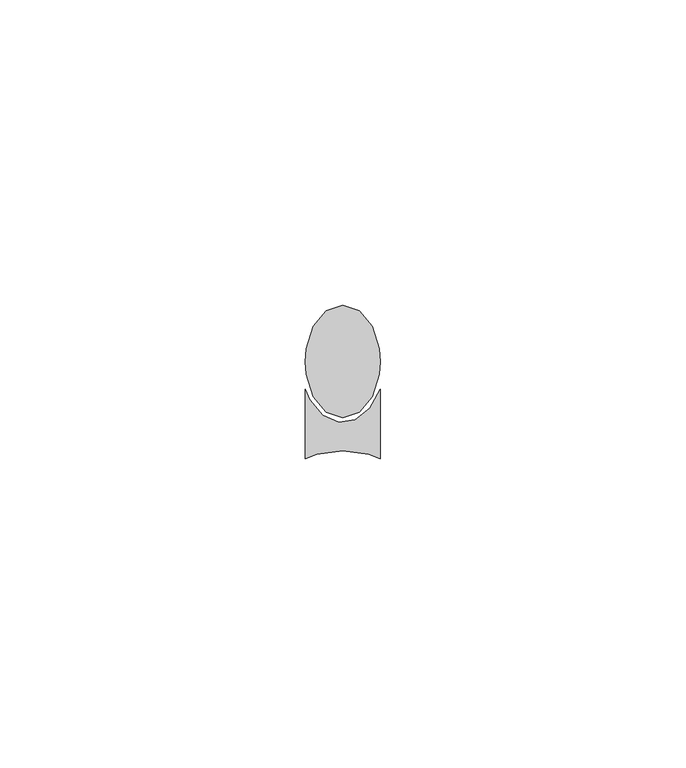
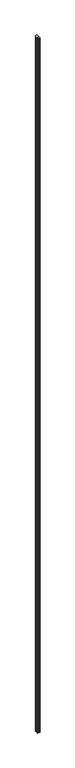
"""IFC4 building model written with IfcOpenShell, lengths in millimetres: proxy geometry, Generic Models 11:Generic Models 1:306267:Generic Models 1:306267 : Generic Models 11:Generic Models 1:306267:300405:Generic Models 1:306267:Generic Models 1:306267 : Generic Models 11:Generic Models 1:306267:300405 : Generic Models 11:Generic Models 1:306267:Generic Models 1:306267 : Generic Models 11:Generic Models 1:306267:300405:11 : Generic Models 11:Generic Models 1:306267:Generic Models 1:306267 : Generic Models 11:Generic Models 1:306267:300405:Generic Models 1:306267:Generic Models 1:306267 : Generic Models 11:Generic Models 1:306267:300405 : Generic Models 11:Generic Models 1:306267:Generic Models 1:306267 : Generic Models 11:Generic Models 1:306267:300405:300182."""

from ifc_helpers import new_model, si_unit, frame, origin, place, context, project, spatial, polyline, outline, extrude, source, transform, mapped, element, save


def generic_models_d67150ab(model_context):
    return source(origin(), model_context, "Body", "SweptSolid", [
        extrude(outline(polyline([(592759.9026632, -579084.0975007), (592755.6213645, -579083.4896058), (592751.3400657, -579084.0975007), (592749.468505, -579084.8288841), (592749.468505, -579073.4570585), (592750.2171531, -579075.1242043), (592752.3168487, -579077.6620411), (592754.9335054, -579078.8254713), (592757.6577712, -579078.4324869), (592760.0634599, -579076.5445668), (592761.7742239, -579073.4570585), (592761.7742239, -579084.8288841), (592759.9026632, -579084.0975007)])), frame((0.0, 0.0, 31.75), z_axis=(0.0, 0.0, 1.0), x_axis=(1.0, 0.0, 0.0)), (0.0, 0.0, 1.0), 3663.95),
        extrude(outline(polyline([(592752.9517388, -579077.1918668), (592750.8108652, -579074.6309323), (592749.62277, -579070.9302746), (592749.468505, -579068.8765646), (592749.62277, -579066.8228545), (592750.8108652, -579063.1221968), (592752.9517388, -579060.5612623), (592755.6213645, -579059.6472753), (592758.2909901, -579060.5612623), (592760.4318637, -579063.1221968), (592761.6199589, -579066.8228545), (592761.7742239, -579068.8765646), (592761.6199589, -579070.9302746), (592760.4318637, -579074.6309323), (592758.2909901, -579077.1918668), (592755.6213645, -579078.1058538), (592752.9517388, -579077.1918668)])), frame((0.0, 0.0, 31.75), z_axis=(0.0, 0.0, 1.0), x_axis=(1.0, 0.0, 0.0)), (0.0, 0.0, 1.0), 3663.95),
    ])


if __name__ == "__main__":
    model = new_model("IFC4")
    model_context = context("Model", 3, world=origin())
    ifc_project = project(units=[si_unit("LENGTHUNIT", "METRE", prefix="MILLI")], contexts=[model_context])
    site = spatial("IfcSite", under=ifc_project)
    building = spatial("IfcBuilding", under=site)
    placement = place(None, origin())
    generic_models_shape = generic_models_d67150ab(model_context)
    element("IfcBuildingElementProxy", 1, Name="Generic Models 11:Generic Models 1:306267:Generic Models 1:306267 : Generic Models 11:Generic Models 1:306267:300405:Generic Models 1:306267:Generic Models 1:306267 : Generic Models 11:Generic Models 1:306267:300405 : Generic Models 11:Generic Models 1:306267:Generic Models 1:306267 : Generic Models 11:Generic Models 1:306267:300405:11 : Generic Models 11:Generic Models 1:306267:Generic Models 1:306267 : Generic Models 11:Generic Models 1:306267:300405:Generic Models 1:306267:Generic Models 1:306267 : Generic Models 11:Generic Models 1:306267:300405 : Generic Models 11:Generic Models 1:306267:Generic Models 1:306267 : Generic Models 11:Generic Models 1:306267:300405:300182", ObjectType="Generic Models 11:Generic Models 1:306267:Generic Models 1:306267 : Generic Models 11:Generic Models 1:306267:300405:Generic Models 1:306267:Generic Models 1:306267 : Generic Models 11:Generic Models 1:306267:300405 : Generic Models 11:Generic Models 1:306267:Generic Models 1:306267 : Generic Models 11:Generic Models 1:306267:300405:11 : Generic Models 11:Generic Models 1:306267:Generic Models 1:306267 : Generic Models 11:Generic Models 1:306267:300405:Generic Models 1:306267:Generic Models 1:306267 : Generic Models 11:Generic Models 1:306267:300405 : Generic Models 11:Generic Models 1:306267:Generic Models 1:306267 : Generic Models 11:Generic Models 1:306267:300405:300182", at=placement, inside=building, context=model_context, shape_type="MappedRepresentation", body=[
        mapped(generic_models_shape, transform((0.0, 0.0, 0.0), x_axis=(1.0, 0.0, 0.0), y_axis=(0.0, 1.0, 0.0), z_axis=(0.0, 0.0, 1.0))),
    ])
    save(model, "model.ifc")

# Revit data of these elements
# Type "Generic Models 11:Generic Models 1:306267:Generic Models 1:306267 : Generic Models 11:Generic Models 1:306267:300405:Generic Models 1:306267:Generic Models 1:306267 : Generic Models 11:Generic Models 1:306267:300405 : Generic Models 11:Generic Models 1:306267:Generic Models 1:306267 : Generic Models 11:Generic Models 1:306267:300405:11 : Generic Models 11:Generic Models 1:306267:Generic Models 1:306267 : Generic Models 11:Generic Models 1:306267:300405:Generic Models 1:306267:Generic Models 1:306267 : Generic Models 11:Generic Models 1:306267:300405 : Generic Models 11:Generic Models 1:306267:Generic Models 1:306267 : Generic Models 11:Generic Models 1:306267:300405:300182"
#   NameOverride = "Generic Models 11:Generic Models 1:306267:Generic Models 1:306267 : Generic Models 11:Generic Models 1:306267:300405:Generic Models 1:306267:Generic Models 1:306267 : Generic Models 11:Generic Models 1:306267:300405 : Generic Models 11:Generic Models 1:306267:Generic Models 1:306267 : Generic Models 11:Generic Models 1:306267:300405:300182"
#   ObjectTypeOverride = "Generic Models 1:306267:Generic Models 1:306267 : Generic Models 11:Generic Models 1:306267:300405 : Generic Models 11:Generic Models 1:306267:Generic Models 1:306267 : Generic Models 11:Generic Models 1:306267:300405"
#   Reference = "Generic Models 1"
#   Tag = "300182"
# Element 1 (IfcBuildingElementProxy, "Generic Models 11:Generic Models 1:306267:Generic Models 1:306267 : Generic Models 11:Generic Models 1:306267:300405:Generic Models 1:306267:Generic Models 1:306267 : Generic Models 11:Generic Models 1:306267:300405 : Generic Models 11:Generic Models 1:306267:Generic Models 1:306267 : Generic Models 11:Generic Models 1:306267:300405:11 : Generic Models 11:Generic Models 1:306267:Generic Models 1:306267 : Generic Models 11:Generic Models 1:306267:300405:Generic Models 1:306267:Generic Models 1:306267 : Generic Models 11:Generic Models 1:306267:300405 : Generic Models 11:Generic Models 1:306267:Generic Models 1:306267 : Generic Models 11:Generic Models 1:306267:300405:300182")
#   Materials on its faces: "SEALANT & BACKER ROD, IF NECESSARY"
# Materials
#   "SEALANT & BACKER ROD, IF NECESSARY": class "Unassigned", colour RGB 120 120 120, transparency 0, Cost = 0
